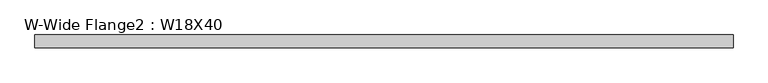
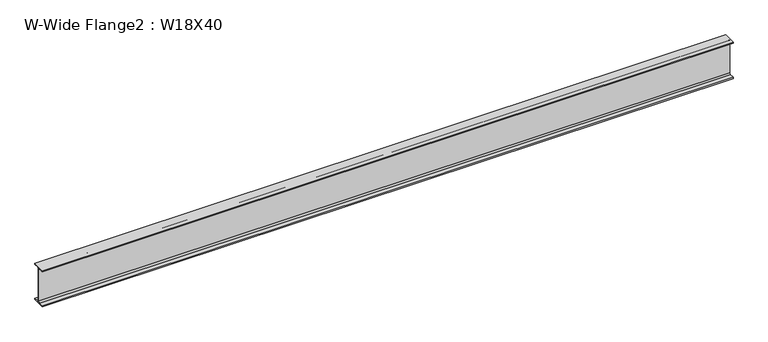
"""IFC4 building model written with IfcOpenShell, lengths in millimetres: beam geometry, W-Wide Flange2 : W18X40."""

from ifc_helpers import new_model, si_unit, point, frame, frame_2d, origin, place, context, project, spatial, polyline, circle_curve, trimmed, segment, composite_curve, outline, extrude, source, transform, mapped, element, save


def w_wide_flange2_w18x40_2ea4b68e(model_context):
    return source(origin(), model_context, "Body", "SweptSolid", [
        extrude(outline(composite_curve([segment(polyline([(76.454, -213.995), (76.454, -227.33), (-76.454, -227.33), (-76.454, -213.995), (-20.828, -213.995)]), True, "CONTINUOUS"), segment(trimmed(circle_curve(frame_2d((-20.828, -197.1675)), 16.8275), [point((-20.828, -213.995))], [point((-4.0005, -197.1675))], True, "CARTESIAN"), True, "CONTINUOUS"), segment(polyline([(-4.0005, -197.1675), (-4.0005, 197.1675)]), True, "CONTINUOUS"), segment(trimmed(circle_curve(frame_2d((-20.828, 197.1675)), 16.8275), [point((-4.0005, 197.1675))], [point((-20.828, 213.995))], True, "CARTESIAN"), True, "CONTINUOUS"), segment(polyline([(-20.828, 213.995), (-76.454, 213.995), (-76.454, 227.33), (76.454, 227.33), (76.454, 213.995), (20.828, 213.995)]), True, "CONTINUOUS"), segment(trimmed(circle_curve(frame_2d((20.828, 197.1675)), 16.8275), [point((20.828, 213.995))], [point((4.0005, 197.1675))], True, "CARTESIAN"), True, "CONTINUOUS"), segment(polyline([(4.0005, 197.1675), (4.0005, -197.1675)]), True, "CONTINUOUS"), segment(trimmed(circle_curve(frame_2d((20.828, -197.1675)), 16.8275), [point((4.0005, -197.1675))], [point((20.828, -213.995))], True, "CARTESIAN"), True, "CONTINUOUS"), segment(polyline([(20.828, -213.995), (76.454, -213.995)]), True, "CONTINUOUS")], self_intersect=False)), frame((-4100.5125, 0.0, 0.0), z_axis=(1.0, 0.0, 0.0), x_axis=(0.0, 1.0, 0.0)), (0.0, 0.0, 1.0), 8201.025),
    ])


if __name__ == "__main__":
    model = new_model("IFC4")
    model_context = context("Model", 3, world=origin())
    ifc_project = project(units=[si_unit("LENGTHUNIT", "METRE", prefix="MILLI")], contexts=[model_context])
    site = spatial("IfcSite", under=ifc_project)
    building = spatial("IfcBuilding", under=site)
    placement = place(None, origin())
    w_wide_flange2_w18x40_shape = w_wide_flange2_w18x40_2ea4b68e(model_context)
    element("IfcBeam", 1, ObjectType="W-Wide Flange2 : W18X40", at=placement, inside=building, context=model_context, shape_type="MappedRepresentation", body=[
        mapped(w_wide_flange2_w18x40_shape, transform((0.0, 0.0, 0.0), x_axis=(1.0, 0.0, 0.0), y_axis=(0.0, 1.0, 0.0), z_axis=(0.0, 0.0, 1.0))),
    ])
    save(model, "model.ifc")

# Revit data of these elements
# Type "W-Wide Flange2 : W18X40"
#   Assembly Code = "B10"
#   W = 40
#   Length [instance default] = 5' - 0"
#   bf = 0' - 6.02"
#   d = 1' - 5.9"
#   k = 0' - 1 3/16"
#   k2 = 0' - 0.6625"
#   tf = 0' - 0.525"
#   tw = 0' - 0.315"
#   A = 0.0819444 SF
#   Structural Material [instance default] = Steel ASTM A992
# Element 1 (IfcBeam, "W-Wide Flange2 : W18X40")
#   Materials on its faces: "Steel ASTM A992"
# Materials
#   "Steel ASTM A992": class "Metal", colour RGB 199 199 199, transparency 0, Description = "Structural steel 50ksi", Cost = 0
